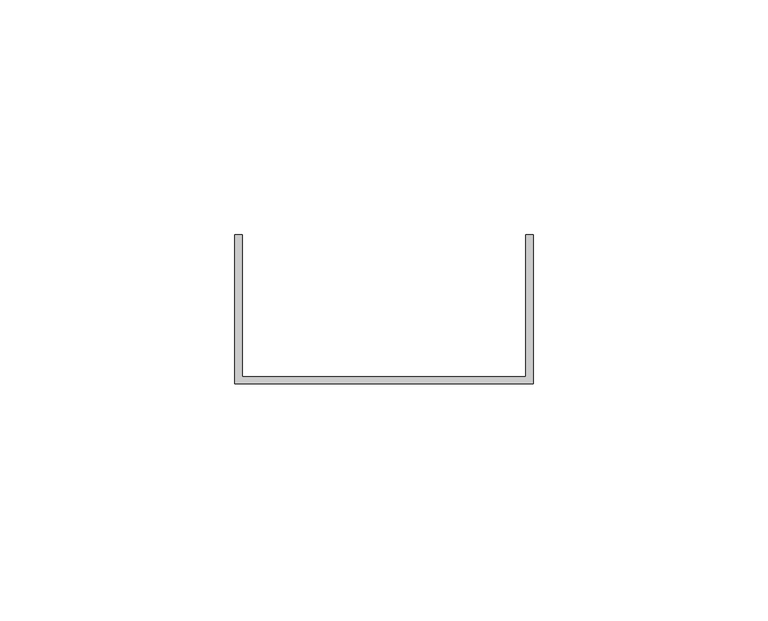
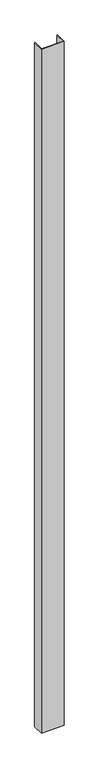
"""IFC4 building model written with IfcOpenShell, lengths in millimetres: proxy geometry, Generic Models 7:Generic Models 1:3:Generic Models 1:3 : Generic Models 7:Generic Models 1:305549:3:Generic Models 1:3:Generic Models 1:3 : Generic Models 7:Generic Models 1:305549:3 : Generic Models 7:Generic Models 1:3:Generic Models 1:3 : Generic Models 7:Generic Models 1:305549:301244:27 : Generic Models 7:Generic Models 1:3:Generic Models 1:3 : Generic Models 7:Generic Models 1:305549:3:Generic Models 1:3:Generic Models 1:3 : Generic Models 7:Generic Models 1:305549:3 : Generic Models 7:Generic Models 1:3:Generic Models 1:3 : Generic Models 7:Generic Models 1:305549:301244:308848."""

import ifcopenshell
import ifcopenshell.guid

model = None  # the IFC model being written
_history = None  # IfcOwnerHistory: only IFC2X3 demands one
_inside = {}  # id of a spatial element -> (the spatial element, [elements in it])
_under = {}  # id of a project, library or spatial element -> (it, [spatial elements below it])
_declared = {}  # id of a project -> (the project, [libraries it declares])
_typed = {}  # id of a type object -> (the type object, [elements of that type])
_made_of = {}  # id of a material, layer set ... -> (it, [elements and type objects made of it])


def new_model(schema):
    """Start an empty IFC model of exactly this schema.

    Asked for "IFC4X3", IfcOpenShell would pick the latest addendum, in which some entities
    have other attributes; the version numbers below select the first issue.
    IFC2X3 requires an IfcOwnerHistory on every rooted entity: one is made here for all.
    """
    global model, _history
    if schema == "IFC4X3":
        model = ifcopenshell.file(schema_version=(4, 3, 0, 0))
    else:
        model = ifcopenshell.file(schema=schema)
    _inside.clear()
    _under.clear()
    _declared.clear()
    _typed.clear()
    _made_of.clear()
    _history = None
    if model.schema == "IFC2X3":
        org = make("IfcOrganization", Name="unknown")
        user = make(
            "IfcPersonAndOrganization",
            ThePerson=make("IfcPerson", FamilyName="unknown"),
            TheOrganization=org,
        )
        app = make(
            "IfcApplication",
            ApplicationDeveloper=org,
            Version="unknown",
            ApplicationFullName="unknown",
            ApplicationIdentifier="unknown",
        )
        _history = make(
            "IfcOwnerHistory",
            OwningUser=user,
            OwningApplication=app,
            ChangeAction="ADDED",
            CreationDate=0,
        )
    return model


def make(cls, **values):
    """One entity of the class cls with the attributes given. An attribute that is None is left unset."""
    return model.create_entity(
        cls, **{name: value for name, value in values.items() if value is not None}
    )


def rooted(cls, **values):
    """An entity with a GlobalId (a new one), such as an element, a storey or a relation."""
    return make(cls, GlobalId=ifcopenshell.guid.new(), OwnerHistory=_history, **values)


def si_unit(unit_type, name, prefix=None):
    """IfcSIUnit, for example si_unit("LENGTHUNIT", "METRE", prefix="MILLI")."""
    return make("IfcSIUnit", UnitType=unit_type, Prefix=prefix, Name=name)


def assignment(units):
    """IfcUnitAssignment: the units of a project."""
    return None if units is None else make("IfcUnitAssignment", Units=units)


def point(xyz):
    """IfcCartesianPoint."""
    return None if xyz is None else make("IfcCartesianPoint", Coordinates=xyz)


def direction(xyz):
    """IfcDirection."""
    return None if xyz is None else make("IfcDirection", DirectionRatios=xyz)


def frame(location, z_axis=None, x_axis=None):
    """IfcAxis2Placement3D, a coordinate frame: its origin and axes. An axis left out is left unset."""
    return make(
        "IfcAxis2Placement3D",
        Location=point(location),
        Axis=direction(z_axis),
        RefDirection=direction(x_axis),
    )


def origin():
    """The frame at (0, 0, 0) with its axes left unset."""
    return frame((0.0, 0.0, 0.0))


def place(relative_to, where):
    """IfcLocalPlacement: puts the frame where relative to a parent placement (None: the world)."""
    return make(
        "IfcLocalPlacement", PlacementRelTo=relative_to, RelativePlacement=where
    )


def context(
    kind, dimensions, precision=None, world=None, true_north=None, identifier=None
):
    """IfcGeometricRepresentationContext, for example the 3D "Model" context."""
    return make(
        "IfcGeometricRepresentationContext",
        ContextIdentifier=identifier,
        ContextType=kind,
        CoordinateSpaceDimension=dimensions,
        Precision=precision,
        WorldCoordinateSystem=world,
        TrueNorth=true_north,
    )


def project(units=None, contexts=None):
    """IfcProject with its units and contexts."""
    return rooted(
        "IfcProject",
        Name="project",
        RepresentationContexts=contexts,
        UnitsInContext=assignment(units),
    )


def spatial(cls, under=None, at=None, **own):
    """A site, building, storey or space (cls), placed at a placement, below another one or the project."""
    s = rooted(cls, ObjectPlacement=at, **own)
    if under is not None:
        _under.setdefault(under.id(), (under, []))[1].append(s)
    return s


def polyline(points):
    """IfcPolyline through the points."""
    return make("IfcPolyline", Points=[point(p) for p in points])


def outline(outer, holes=None, kind="AREA"):
    """IfcArbitraryClosedProfileDef: a profile drawn as a closed curve; with holes, ...WithVoids."""
    if holes is None:
        return make("IfcArbitraryClosedProfileDef", ProfileType=kind, OuterCurve=outer)
    return make(
        "IfcArbitraryProfileDefWithVoids",
        ProfileType=kind,
        OuterCurve=outer,
        InnerCurves=holes,
    )


def extrude(swept, where, along, depth):
    """IfcExtrudedAreaSolid: the profile swept, set in the frame where, extruded along a direction by depth."""
    return make(
        "IfcExtrudedAreaSolid",
        SweptArea=swept,
        Position=where,
        ExtrudedDirection=direction(along),
        Depth=depth,
    )


def shape(context_of_items, identifier, shape_type, items):
    """IfcShapeRepresentation: the items that make up one representation, for example the "Body"."""
    return make(
        "IfcShapeRepresentation",
        ContextOfItems=context_of_items,
        RepresentationIdentifier=identifier,
        RepresentationType=shape_type,
        Items=items,
    )


def source(mapping_origin, context_of_items, identifier, shape_type, items):
    """IfcRepresentationMap: a shape defined once, which mapped items show again and again."""
    return make(
        "IfcRepresentationMap",
        MappingOrigin=mapping_origin,
        MappedRepresentation=shape(context_of_items, identifier, shape_type, items),
    )


def transform(
    local_origin,
    x_axis=None,
    y_axis=None,
    z_axis=None,
    scale=None,
    scale2=None,
    scale3=None,
    uniform=True,
):
    """IfcCartesianTransformationOperator3D, or its non-uniform kind. x_axis, y_axis, z_axis: its Axis1, 2, 3."""
    if uniform:
        return make(
            "IfcCartesianTransformationOperator3D",
            Axis1=direction(x_axis),
            Axis2=direction(y_axis),
            LocalOrigin=point(local_origin),
            Scale=scale,
            Axis3=direction(z_axis),
        )
    return make(
        "IfcCartesianTransformationOperator3DnonUniform",
        Axis1=direction(x_axis),
        Axis2=direction(y_axis),
        LocalOrigin=point(local_origin),
        Scale=scale,
        Axis3=direction(z_axis),
        Scale2=scale2,
        Scale3=scale3,
    )


def mapped(mapping_source, mapping_target):
    """IfcMappedItem: shows the shape of a source again, moved by a transform."""
    return make(
        "IfcMappedItem", MappingSource=mapping_source, MappingTarget=mapping_target
    )


def made_of(thing, what):
    """Note that an element or type object is made of a material, layer set ...; save() writes the relation."""
    if what is not None:
        _made_of.setdefault(what.id(), (what, []))[1].append(thing)
    return thing


def element(
    cls,
    number,
    at=None,
    inside=None,
    cuts=None,
    type_object=None,
    material=None,
    context=None,
    identifier="Body",
    shape_type=None,
    held_by="IfcProductDefinitionShape",
    body=None,
    shapes=None,
    **own,
):
    """One element of the class cls, such as IfcWall. Its Tag is "e" and its number.

    at: its placement. inside: the storey or other place that contains it. cuts: it is an
    opening in that element (IfcRelVoidsElement). A single representation is given by context,
    identifier, shape_type and body (its items); several are given by shapes. held_by: the class
    of the entity that holds the representations. save() writes the other relations.
    """
    e = rooted(cls, Tag="e%d" % number, ObjectPlacement=at, **own)
    if body is not None:
        shapes = [shape(context, identifier, shape_type, body)]
    if shapes is not None:
        e.Representation = make(held_by, Representations=shapes)
    if inside is not None:
        _inside.setdefault(inside.id(), (inside, []))[1].append(e)
    if cuts is not None:
        rooted(
            "IfcRelVoidsElement", RelatingBuildingElement=cuts, RelatedOpeningElement=e
        )
    if type_object is not None:
        _typed.setdefault(type_object.id(), (type_object, []))[1].append(e)
    return made_of(e, material)


def aggregate(whole, parts):
    """IfcRelAggregates: a whole, such as a stair, and the parts it consists of."""
    return rooted("IfcRelAggregates", RelatingObject=whole, RelatedObjects=parts)


def save(model, path):
    """Write the relations noted so far, then the file.

    IfcRelAggregates (storeys below a building ...), IfcRelContainedInSpatialStructure (elements
    in a storey), IfcRelDefinesByType, IfcRelAssociatesMaterial and IfcRelDeclares: one each for
    every whole, place, type object, material and project.
    """
    for whole, parts in _under.values():
        aggregate(whole, parts)
    for where, things in _inside.values():
        rooted(
            "IfcRelContainedInSpatialStructure",
            RelatedElements=things,
            RelatingStructure=where,
        )
    for kind, things in _typed.values():
        rooted("IfcRelDefinesByType", RelatedObjects=things, RelatingType=kind)
    for what, things in _made_of.values():
        rooted("IfcRelAssociatesMaterial", RelatedObjects=things, RelatingMaterial=what)
    for by, libraries in _declared.values():
        rooted("IfcRelDeclares", RelatingContext=by, RelatedDefinitions=libraries)
    model.write(path)


def generic_models_97e3ebf6(model_context):
    return source(origin(), model_context, "Body", "SweptSolid", [
        extrude(outline(polyline([(560340.2617239, -572587.1913841), (560276.7617239, -572587.1913841), (560276.7617239, -572555.4413841), (560278.3492239, -572555.4413841), (560278.3492239, -572585.6038841), (560338.6742239, -572585.6038841), (560338.6742239, -572555.4413841), (560340.2617239, -572555.4413841), (560340.2617239, -572587.1913841)])), frame((0.0, 0.0, 4133.81326), z_axis=(0.0, 0.0, 1.0), x_axis=(1.0, 0.0, 0.0)), (0.0, 0.0, 1.0), 2000.28674),
    ])


if __name__ == "__main__":
    model = new_model("IFC4")
    model_context = context("Model", 3, world=origin())
    ifc_project = project(units=[si_unit("LENGTHUNIT", "METRE", prefix="MILLI")], contexts=[model_context])
    site = spatial("IfcSite", under=ifc_project)
    building = spatial("IfcBuilding", under=site)
    placement = place(None, origin())
    generic_models_shape = generic_models_97e3ebf6(model_context)
    element("IfcBuildingElementProxy", 1, Name="Generic Models 7:Generic Models 1:3:Generic Models 1:3 : Generic Models 7:Generic Models 1:305549:3:Generic Models 1:3:Generic Models 1:3 : Generic Models 7:Generic Models 1:305549:3 : Generic Models 7:Generic Models 1:3:Generic Models 1:3 : Generic Models 7:Generic Models 1:305549:301244:27 : Generic Models 7:Generic Models 1:3:Generic Models 1:3 : Generic Models 7:Generic Models 1:305549:3:Generic Models 1:3:Generic Models 1:3 : Generic Models 7:Generic Models 1:305549:3 : Generic Models 7:Generic Models 1:3:Generic Models 1:3 : Generic Models 7:Generic Models 1:305549:301244:308848", ObjectType="Generic Models 7:Generic Models 1:3:Generic Models 1:3 : Generic Models 7:Generic Models 1:305549:3:Generic Models 1:3:Generic Models 1:3 : Generic Models 7:Generic Models 1:305549:3 : Generic Models 7:Generic Models 1:3:Generic Models 1:3 : Generic Models 7:Generic Models 1:305549:301244:27 : Generic Models 7:Generic Models 1:3:Generic Models 1:3 : Generic Models 7:Generic Models 1:305549:3:Generic Models 1:3:Generic Models 1:3 : Generic Models 7:Generic Models 1:305549:3 : Generic Models 7:Generic Models 1:3:Generic Models 1:3 : Generic Models 7:Generic Models 1:305549:301244:308848", at=placement, inside=building, context=model_context, shape_type="MappedRepresentation", body=[
        mapped(generic_models_shape, transform((0.0, 0.0, 0.0), x_axis=(1.0, 0.0, 0.0), y_axis=(0.0, 1.0, 0.0), z_axis=(0.0, 0.0, 1.0))),
    ])
    save(model, "model.ifc")

# Revit data of these elements
# Type "Generic Models 7:Generic Models 1:3:Generic Models 1:3 : Generic Models 7:Generic Models 1:305549:3:Generic Models 1:3:Generic Models 1:3 : Generic Models 7:Generic Models 1:305549:3 : Generic Models 7:Generic Models 1:3:Generic Models 1:3 : Generic Models 7:Generic Models 1:305549:301244:27 : Generic Models 7:Generic Models 1:3:Generic Models 1:3 : Generic Models 7:Generic Models 1:305549:3:Generic Models 1:3:Generic Models 1:3 : Generic Models 7:Generic Models 1:305549:3 : Generic Models 7:Generic Models 1:3:Generic Models 1:3 : Generic Models 7:Generic Models 1:305549:301244:308848"
#   NameOverride = "Generic Models 7:Generic Models 1:3:Generic Models 1:3 : Generic Models 7:Generic Models 1:305549:3:Generic Models 1:3:Generic Models 1:3 : Generic Models 7:Generic Models 1:305549:3 : Generic Models 7:Generic Models 1:3:Generic Models 1:3 : Generic Models 7:Generic Models 1:305549:301244:308848"
#   ObjectTypeOverride = "Generic Models 1:3:Generic Models 1:3 : Generic Models 7:Generic Models 1:305549:3 : Generic Models 7:Generic Models 1:3:Generic Models 1:3 : Generic Models 7:Generic Models 1:305549:301244"
#   Reference = "Generic Models 1"
#   Tag = "308848"
# Element 1 (IfcBuildingElementProxy, "Generic Models 7:Generic Models 1:3:Generic Models 1:3 : Generic Models 7:Generic Models 1:305549:3:Generic Models 1:3:Generic Models 1:3 : Generic Models 7:Generic Models 1:305549:3 : Generic Models 7:Generic Models 1:3:Generic Models 1:3 : Generic Models 7:Generic Models 1:305549:301244:27 : Generic Models 7:Generic Models 1:3:Generic Models 1:3 : Generic Models 7:Generic Models 1:305549:3:Generic Models 1:3:Generic Models 1:3 : Generic Models 7:Generic Models 1:305549:3 : Generic Models 7:Generic Models 1:3:Generic Models 1:3 : Generic Models 7:Generic Models 1:305549:301244:308848")
#   Materials on its faces: "GALVANIZED U-CHANNEL (250T125-33)"
# Materials
#   "GALVANIZED U-CHANNEL (250T125-33)": class "Unassigned", colour RGB 202 201 200, transparency 0, Keynote = "M05451300.02", Cost = 0
